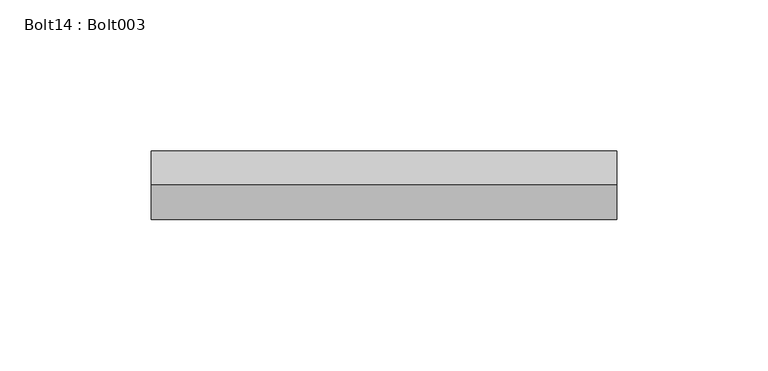
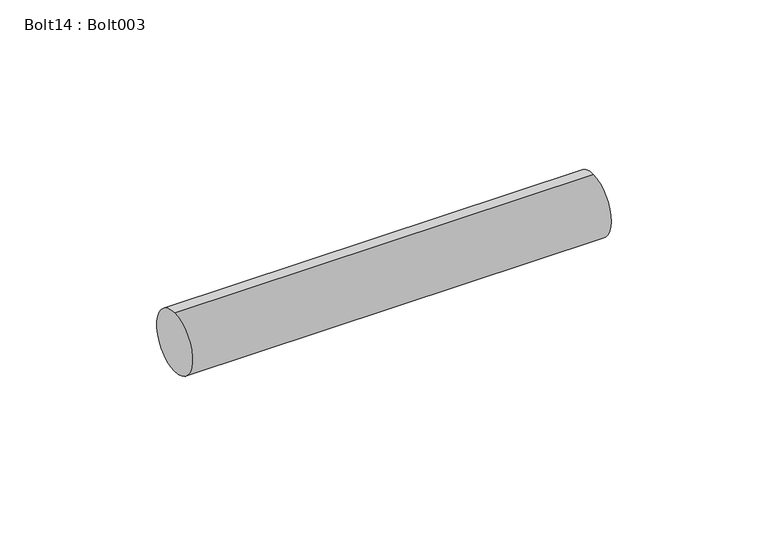
"""IFC4 building model written with IfcOpenShell, lengths in millimetres: proxy geometry, Bolt14 : Bolt003."""

from ifc_helpers import new_model, si_unit, point, frame, frame_2d, origin, place, context, project, spatial, circle_curve, trimmed, segment, composite_curve, outline, extrude, source, transform, mapped, element, save


def bolt14_bolt003_cd8d5e77(model_context):
    return source(origin(), model_context, "Body", "SweptSolid", [
        extrude(outline(composite_curve([segment(trimmed(circle_curve(frame_2d((1896.5882072, 40070.0545241)), 11.4045168), [point((1896.5882072, 40058.6500073))], [point((1896.5882072, 40081.4590409))], False, "CARTESIAN"), True, "CONTINUOUS"), segment(trimmed(circle_curve(frame_2d((1896.5882072, 40070.0545241)), 11.4045168), [point((1896.5882072, 40081.4590409))], [point((1896.5882072, 40058.6500073))], False, "CARTESIAN"), True, "CONTINUOUS")], self_intersect=False)), frame((10287.3140827, 0.0, 0.0), z_axis=(1.0, 0.0, 0.0), x_axis=(0.0, 1.0, 0.0)), (0.0, 0.0, 1.0), 154.0602393),
    ])


if __name__ == "__main__":
    model = new_model("IFC4")
    model_context = context("Model", 3, world=origin())
    ifc_project = project(units=[si_unit("LENGTHUNIT", "METRE", prefix="MILLI")], contexts=[model_context])
    site = spatial("IfcSite", under=ifc_project)
    building = spatial("IfcBuilding", under=site)
    placement = place(None, origin())
    bolt14_bolt003_shape = bolt14_bolt003_cd8d5e77(model_context)
    element("IfcBuildingElementProxy", 1, Name="Bolt14 : Bolt003", ObjectType="Bolt14 : Bolt003", at=placement, inside=building, context=model_context, shape_type="MappedRepresentation", body=[
        mapped(bolt14_bolt003_shape, transform((0.0, 0.0, 0.0), x_axis=(1.0, 0.0, 0.0), y_axis=(0.0, 1.0, 0.0), z_axis=(0.0, 0.0, 1.0))),
    ])
    save(model, "model.ifc")

# Revit data of these elements
# Type "Bolt14 : Bolt003"
#   NameOverride = "Bolt003"
# Element 1 (IfcBuildingElementProxy, "Bolt14 : Bolt003")
#   Materials on its faces: "TUBE STEEL STRINGER WELDED TO ANCHORED STEEL PLATE - SEE STRUCT DWGS"
# Materials
#   "TUBE STEEL STRINGER WELDED TO ANCHORED STEEL PLATE - SEE STRUCT DWGS": class "Unassigned", colour RGB 128 128 128, transparency 0, Cost = 0
